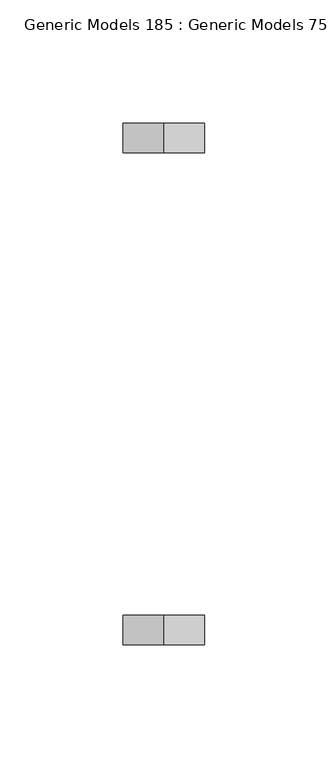
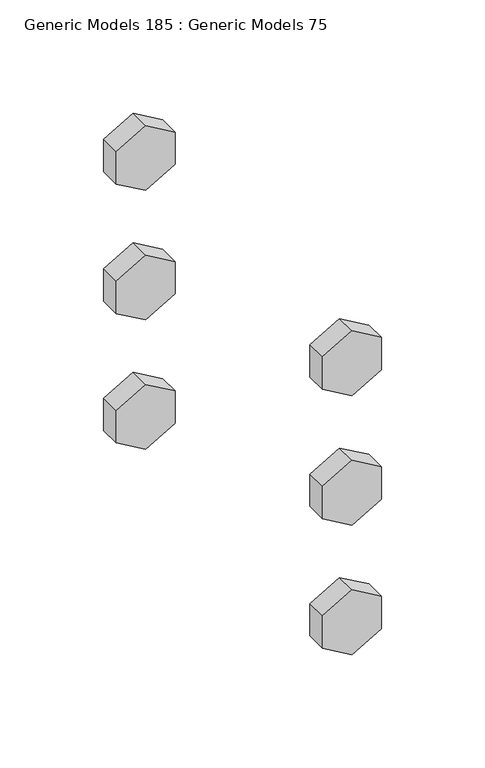
"""IFC4 building model written with IfcOpenShell, lengths in millimetres: proxy geometry, Generic Models 185 : Generic Models 75."""

from ifc_helpers import new_model, si_unit, frame, origin, place, context, project, spatial, polyline, outline, extrude, source, transform, mapped, element, save


def generic_models_185_generic_models_75_26c2082f(model_context):
    return source(origin(), model_context, "Body", "SweptSolid", [
        extrude(outline(polyline([(269043.15, 31689.0368192), (269033.625, 31705.5346032), (269043.15, 31722.0323871), (269062.2, 31722.0323871), (269071.725, 31705.5346032), (269062.2, 31689.0368192), (269043.15, 31689.0368192)])), frame((0.0, 30868.0031612, 0.0), z_axis=(0.0, 1.0, 0.0), x_axis=(0.0, 0.0, 1.0)), (0.0, 0.0, 1.0), 11.90625),
        extrude(outline(polyline([(268966.95, 31689.0368192), (268957.425, 31705.5346032), (268966.95, 31722.0323871), (268986.0, 31722.0323871), (268995.525, 31705.5346032), (268986.0, 31689.0368192), (268966.95, 31689.0368192)])), frame((0.0, 30868.0031612, 0.0), z_axis=(0.0, 1.0, 0.0), x_axis=(0.0, 0.0, 1.0)), (0.0, 0.0, 1.0), 11.90625),
        extrude(outline(polyline([(268890.75, 31689.0368192), (268881.225, 31705.5346032), (268890.75, 31722.0323871), (268909.8, 31722.0323871), (268919.325, 31705.5346032), (268909.8, 31689.0368192), (268890.75, 31689.0368192)])), frame((0.0, 30868.0031612, 0.0), z_axis=(0.0, 1.0, 0.0), x_axis=(0.0, 0.0, 1.0)), (0.0, 0.0, 1.0), 11.90625),
        extrude(outline(polyline([(269043.15, 31689.0368192), (269033.625, 31705.5346032), (269043.15, 31722.0323871), (269062.2, 31722.0323871), (269071.725, 31705.5346032), (269062.2, 31689.0368192), (269043.15, 31689.0368192)])), frame((0.0, 30668.7719112, 0.0), z_axis=(0.0, 1.0, 0.0), x_axis=(0.0, 0.0, 1.0)), (0.0, 0.0, 1.0), 11.90625),
        extrude(outline(polyline([(268966.95, 31689.0368192), (268957.425, 31705.5346032), (268966.95, 31722.0323871), (268986.0, 31722.0323871), (268995.525, 31705.5346032), (268986.0, 31689.0368192), (268966.95, 31689.0368192)])), frame((0.0, 30668.7719112, 0.0), z_axis=(0.0, 1.0, 0.0), x_axis=(0.0, 0.0, 1.0)), (0.0, 0.0, 1.0), 11.90625),
        extrude(outline(polyline([(268890.75, 31689.0368192), (268881.225, 31705.5346032), (268890.75, 31722.0323871), (268909.8, 31722.0323871), (268919.325, 31705.5346032), (268909.8, 31689.0368192), (268890.75, 31689.0368192)])), frame((0.0, 30668.7719112, 0.0), z_axis=(0.0, 1.0, 0.0), x_axis=(0.0, 0.0, 1.0)), (0.0, 0.0, 1.0), 11.90625),
    ])


if __name__ == "__main__":
    model = new_model("IFC4")
    model_context = context("Model", 3, world=origin())
    ifc_project = project(units=[si_unit("LENGTHUNIT", "METRE", prefix="MILLI")], contexts=[model_context])
    site = spatial("IfcSite", under=ifc_project)
    building = spatial("IfcBuilding", under=site)
    placement = place(None, origin())
    generic_models_185_generic_models_75_shape = generic_models_185_generic_models_75_26c2082f(model_context)
    element("IfcBuildingElementProxy", 1, Name="Generic Models 185 : Generic Models 75", ObjectType="Generic Models 185 : Generic Models 75", at=placement, inside=building, context=model_context, shape_type="MappedRepresentation", body=[
        mapped(generic_models_185_generic_models_75_shape, transform((0.0, 0.0, 0.0), x_axis=(1.0, 0.0, 0.0), y_axis=(0.0, 1.0, 0.0), z_axis=(0.0, 0.0, 1.0))),
    ])
    save(model, "model.ifc")
